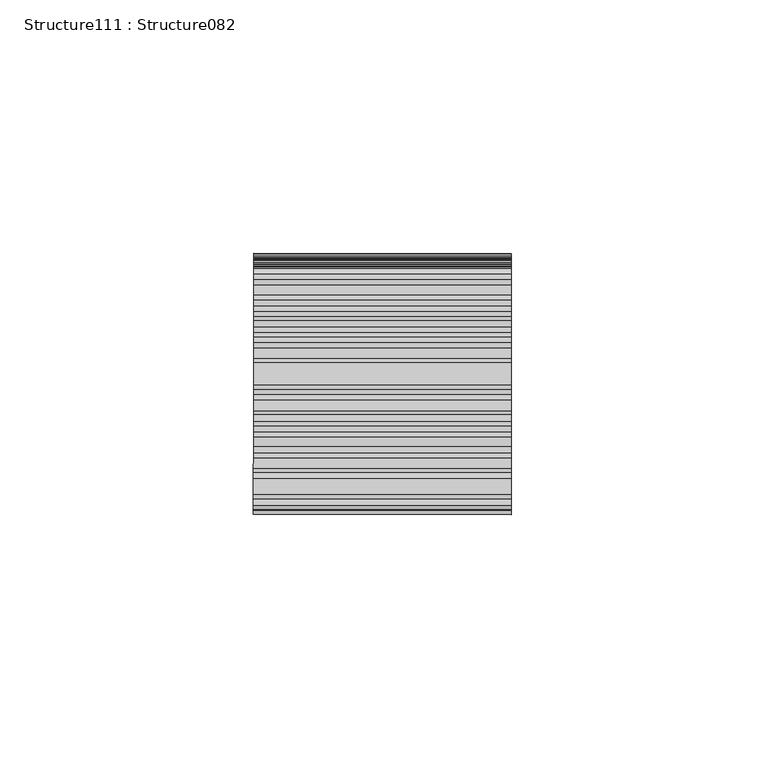
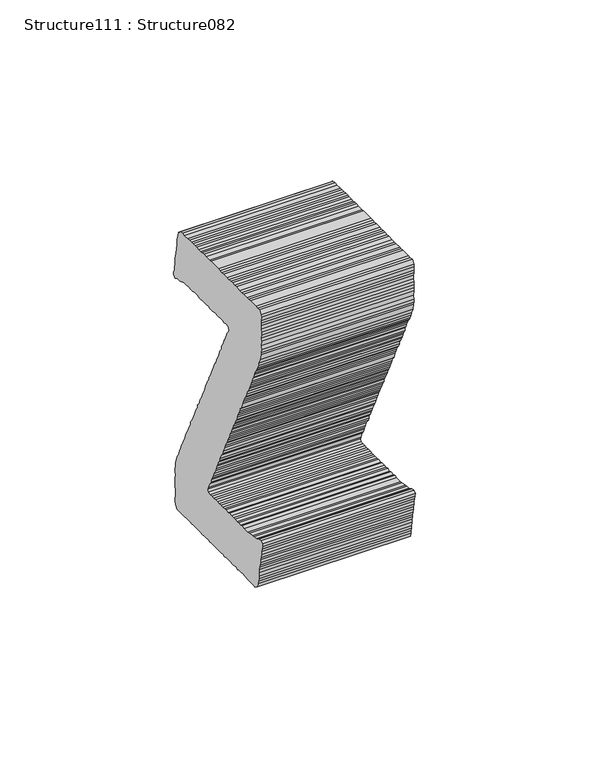
"""IFC4 building model written with IfcOpenShell, lengths in millimetres: proxy geometry, Structure111 : Structure082."""

from ifc_helpers import new_model, si_unit, frame, origin, place, context, project, spatial, polyline, outline, extrude, source, transform, mapped, element, save


def structure111_structure082_6162c2b4(model_context):
    return source(origin(), model_context, "Body", "SweptSolid", [
        extrude(outline(polyline([(1.0465822, 0.0), (1.5142605, -1.0826543), (1.8028074, -2.1135614), (2.0909573, -3.1430563), (2.6061462, -4.0449015), (2.8502721, -5.2548528), (3.1872117, -6.1093644), (3.6556847, -7.1891061), (3.9440992, -8.2204986), (4.2203696, -8.9609175), (4.5094019, -9.991957), (4.9126595, -10.9618421), (5.4428175, -12.1509985), (5.8937621, -12.9403834), (6.1859717, -13.9741156), (6.525074, -14.8273918), (6.9391965, -16.0824248), (6.1536508, -17.5830856), (5.2962264, -17.9192304), (4.5730271, -18.4860339), (2.54318, -19.6456059), (0.6070291, -20.4512831), (-0.1826648, -20.9024043), (-1.1334764, -21.5922674), (-2.1003606, -21.9979086), (-2.6463696, -22.610192), (-3.6794394, -22.8999744), (-4.6780705, -23.770823), (-6.7263728, -24.6405679), (-8.417912, -25.6068779), (-9.1900776, -26.3483556), (-10.110996, -26.5740704), (-10.9971667, -27.3806747), (-12.0111634, -27.9599313), (-12.981048, -28.3603202), (-14.6704246, -29.3253948), (-15.7497691, -29.7952802), (-16.411328, -30.4735727), (-17.3300838, -30.698052), (-18.32717, -31.5680181), (-19.2970547, -31.968407), (-20.2482642, -32.6654638), (-21.2144414, -33.0637349), (-24.6003005, -34.9979433), (-25.6624256, -35.7583618), (-26.4039911, -36.028321), (-28.3232316, -37.1247078), (-29.1585823, -37.755579), (-31.7535117, -39.2379603), (-32.947699, -39.7664846), (-34.315767, -39.2051539), (-35.0588773, -38.4294134), (-35.508057, -37.643118), (-35.8622159, -36.4980732), (-36.4931748, -35.658265), (-37.0083637, -34.7564196), (-37.5073921, -34.1432538), (-39.0547236, -31.4346284), (-39.3428734, -30.4051334), (-40.2114716, -29.4097246), (-40.6011726, -28.7275476), (-41.0176342, -27.4734411), (-41.534588, -26.5685062), (-41.9836354, -24.7351432), (-42.0347194, -23.8595277), (-42.032072, -22.81758), (-42.2105855, -21.7188976), (-42.4503427, -20.5130072), (-42.3214126, -19.6878151), (-42.5655385, -18.4778639), (-42.7883853, -17.562683), (-42.547966, -16.6758505), (-42.8533791, -15.3521594), (-42.7910767, -13.3709256), (-43.192084, -12.4042626), (-43.3072797, -10.3691192), (-43.1926575, -9.2627947), (-43.3049853, -8.2799712), (-43.3048528, -7.2329036), (-43.3031756, -6.1849535), (-43.7742525, -5.1042406), (-43.6423219, -4.2843008), (-43.708375, -3.1213743), (-43.770942, -1.9609638), (-43.9511768, 0.1837271), (-44.0597094, 1.1642111), (-44.1739787, 2.150433), (-44.0452698, 2.9709913), (-44.3991199, 4.1162124), (-44.2211359, 5.1116215), (-44.287189, 6.2745479), (-44.5119772, 7.1931272), (-44.5100798, 8.2371053), (-44.5581635, 9.1074684), (-44.7365892, 10.2016932), (-44.6869601, 11.4311143), (-44.8652094, 12.5250302), (-44.9147487, 13.401528), (-45.2062971, 14.4290815), (-45.2025896, 15.4777816), (-45.2685551, 16.6362505), (-45.2040456, 18.6207942), (-45.4739171, 19.3579022), (-45.4921955, 20.6968713), (-45.4305991, 21.6327588), (-45.6538425, 22.5522206), (-45.7675827, 23.534647), (-45.781007, 24.8694228), (-45.898189, 25.8564395), (-46.0723338, 26.951061), (-45.8294877, 27.8343626), (-46.1845292, 28.9809521), (-46.166162, 30.7858781), (-46.2338924, 31.9474367), (-46.58611, 33.0890829), (-46.5859775, 34.1361506), (-46.4099349, 35.134958), (-46.8111186, 36.1019299), (-46.8139866, 37.1542499), (-46.6973341, 38.2613244), (-47.1038577, 39.2297534), (-46.9729862, 40.051547), (-47.1513231, 41.1499204), (-47.1008563, 42.3728537), (-47.2148614, 43.3543093), (-47.1498664, 44.2921383), (-47.1473955, 45.334395), (-48.2286368, 45.9194333), (-49.2612212, 45.6295185), (-50.1475683, 44.823223), (-51.1789169, 44.5340141), (-51.9683019, 44.0830695), (-52.7424976, 43.3408416), (-53.5321915, 42.8897205), (-54.6769273, 42.535738), (-55.2911081, 42.037769), (-56.1252671, 41.4083981), (-57.1426623, 40.8272002), (-58.0612416, 40.6024121), (-58.7875738, 40.0403753), (-59.9155756, 39.3959922), (-60.5251229, 38.8949332), (-62.446217, 37.7974874), (-63.5878633, 37.4452699), (-65.168487, 36.5423216), (-65.9426827, 35.8000938), (-66.7323767, 35.3489726), (-67.9895728, 34.930746), (-68.6497634, 34.2536448), (-70.2285333, 33.3517555), (-71.0991615, 32.2561187), (-71.7582932, 31.5771638), (-72.5988069, 30.9503094), (-73.3209914, 30.3824465), (-73.9700082, 29.4203739), (-75.1444612, 29.6427789), (-75.5472774, 30.6133258), (-75.6599142, 31.5959728), (-75.9491231, 32.6273214), (-76.4825907, 33.8186848), (-76.7563451, 34.5625899), (-77.3979043, 35.6856483), (-77.8037656, 36.6565046), (-77.9611768, 37.4578568), (-78.7208883, 39.5739343), (-78.9457652, 40.4883651), (-79.5289046, 41.5091588), (-79.9296029, 42.4759983), (-80.2196065, 43.5044341), (-80.3809006, 44.3125834), (-80.7963033, 45.5648362), (-80.2833641, 46.7651146), (-79.3967969, 47.567438), (-78.3678311, 47.8593835), (-76.6744382, 48.8267524), (-75.9003312, 49.5648317), (-74.8205456, 50.0325104), (-73.9810907, 50.6612185), (-73.0807902, 51.1755248), (-72.3374587, 51.4510005), (-71.1465806, 51.9846006), (-70.2428816, 52.5008483), (-69.5166819, 53.0623996), (-68.6809344, 53.6889898), (-67.5989861, 54.157904), (-65.7952955, 55.1882817), (-65.1807613, 55.6885014), (-61.3475326, 57.8782746), (-60.4939035, 58.216759), (-59.6394795, 58.558156), (-58.7510585, 59.3615383), (-56.9476768, 60.3917395), (-56.1430139, 60.5555496), (-55.1405878, 61.4240586), (-54.3508938, 61.8751798), (-53.2729619, 62.3417996), (-52.4335071, 62.9705076), (-50.7273077, 63.64933), (-49.598997, 64.2938897), (-48.7584832, 64.9207441), (-46.9551015, 65.9509453), (-46.2165364, 66.2261567), (-45.3265706, 67.0304216), (-42.619181, 68.5770471), (-41.7023666, 68.8049248), (-40.7002495, 69.6732574), (-39.441156, 69.0422977), (-38.8785454, 68.3171129), (-38.4091899, 67.2358265), (-37.9608926, 66.4510759), (-37.5601943, 65.4842364), (-36.9770549, 64.4634427), (-36.3017187, 63.8063416), (-35.7874124, 62.9060412), (-35.3152329, 61.8198115), (-34.6912021, 60.9871096), (-34.0795369, 59.3912967), (-33.2721824, 58.5030958), (-32.8024739, 57.4211915), (-32.5329114, 56.6839071), (-31.9022618, 54.7944715), (-31.7914347, 52.7633889), (-31.3883969, 51.8003446), (-31.3716192, 50.4596987), (-31.325168, 49.5929106), (-31.4349369, 48.4766555), (-31.3239773, 47.4926405), (-31.3219471, 46.4468083), (-31.0344151, 45.4169606), (-31.2123991, 44.4215517), (-30.8094504, 43.4514902), (-30.7909955, 42.1122121), (-30.6298339, 41.3035774), (-30.5666487, 40.1463887), (-30.5193598, 39.2731128), (-30.3897237, 38.0039048), (-30.6341146, 37.1197207), (-30.2926298, 36.2608393), (-30.1667452, 34.9903078), (-30.3430967, 33.9913238), (-30.2305924, 33.0081913), (-30.0513729, 31.9082732), (-29.9881437, 30.75029), (-29.5864745, 28.7366035), (-29.9428402, 27.7880427), (-29.6508071, 26.7546195), (-29.5383027, 25.7714871), (-29.5217893, 24.4356076), (-29.3610687, 23.6291797), (-29.1849822, 22.5340284), (-29.2968693, 21.4186121), (-29.1362365, 20.6166416), (-29.1379137, 19.5686915), (-29.1378697, 18.5213149), (-28.9575026, 17.4236916), (-29.0713311, 16.3116737), (-28.7347005, 15.4569856), (-28.8321922, 14.0559796), (-28.6061681, 13.1381062), (-28.6037413, 12.0879931), (-28.5396295, 10.9284651), (-28.4291554, 9.9445826), (-28.4934432, 9.0141239), (-28.2506856, 7.8029812), (-28.2523628, 6.7550311), (-28.0406459, 5.0774452), (-27.8501639, 3.6967041), (-27.960992, 2.5794341), (-27.8484876, 0.5497195), (-27.5760125, -0.1883598), (-27.737086, -1.4744784), (-27.5113276, -2.39906), (-27.6234349, -3.5105042), (-27.2208829, -4.4762847), (-27.1102323, -5.4604761), (-27.2860984, -7.5061747), (-27.0463411, -8.7120651), (-26.9794055, -9.8765364), (-26.9807737, -10.9243099), (-26.6402592, -11.7771891), (-26.8049077, -13.0649401), (-26.5800755, -15.030896), (-26.4152953, -15.8415612), (-25.805439, -16.386908), (-24.7258299, -15.9189204), (-23.7725024, -15.225571), (-22.9187408, -14.8866013), (-22.0190581, -14.3726479), (-21.0669665, -13.6800045), (-20.1457834, -13.4561876), (-19.3116685, -12.8260224), (-18.5667046, -12.5541218), (-17.6188935, -11.8590065), (-16.8917225, -11.2948514), (-15.6331584, -10.878302), (-15.0864871, -10.2635913), (-14.0084227, -9.7964862), (-13.1047237, -9.2802384), (-12.2672551, -8.6530746), (-11.2348474, -8.3657195), (-10.6241084, -7.8631602), (-9.4280673, -7.3335769), (-8.7686267, -6.6544455), (-7.7368371, -6.3674434), (-5.9316016, -5.3361832), (-5.1581559, -4.5919252), (-3.5981502, -3.4003852), (-2.9834395, -2.9004745), (-1.9211379, -2.1403649), (-1.371246, -1.5348784), (-0.8394548, -0.6287082), (0.0, 0.0), (1.0465822, 0.0)])), frame((-56111.2132415, 291928.3025144, -357.1515075), z_axis=(-0.9999998917542983, 0.00046528635450596146, 0.0), x_axis=(-0.00040401088704419266, -0.8683058065241513, -0.4960290950454885)), (0.0, 0.0, 1.0), 50.8),
    ])


if __name__ == "__main__":
    model = new_model("IFC4")
    model_context = context("Model", 3, world=origin())
    ifc_project = project(units=[si_unit("LENGTHUNIT", "METRE", prefix="MILLI")], contexts=[model_context])
    site = spatial("IfcSite", under=ifc_project)
    building = spatial("IfcBuilding", under=site)
    placement = place(None, origin())
    structure111_structure082_shape = structure111_structure082_6162c2b4(model_context)
    element("IfcBuildingElementProxy", 1, Name="Structure111 : Structure082", ObjectType="Structure111 : Structure082", at=placement, inside=building, context=model_context, shape_type="MappedRepresentation", body=[
        mapped(structure111_structure082_shape, transform((0.0, 0.0, 0.0), x_axis=(1.0, 0.0, 0.0), y_axis=(0.0, 1.0, 0.0), z_axis=(0.0, 0.0, 1.0))),
    ])
    save(model, "model.ifc")

# Revit data of these elements
# Type "Structure111 : Structure082"
#   NameOverride = "Structure082"
# Element 1 (IfcBuildingElementProxy, "Structure111 : Structure082")
#   Materials on its faces: "BRUSHED ALUMINUM LETTERING"
# Materials
#   "BRUSHED ALUMINUM LETTERING": class "Unassigned", colour RGB 169 181 186, transparency 0, Cost = 0
